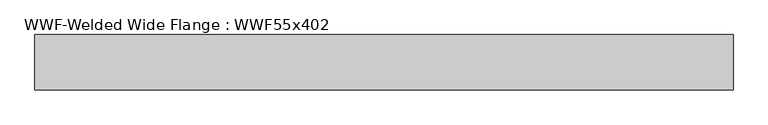
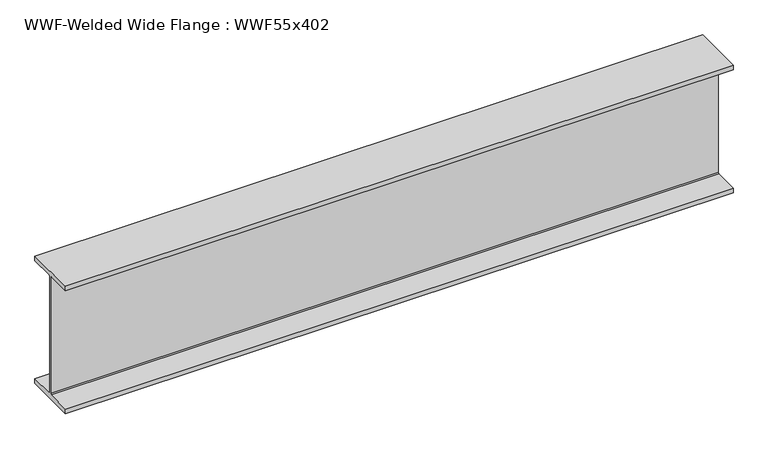
"""IFC4 building model written with IfcOpenShell, lengths in millimetres: beam geometry, WWF-Welded Wide Flange : WWF55x402."""

from ifc_helpers import new_model, si_unit, frame, origin, place, context, project, spatial, polyline, outline, extrude, source, transform, mapped, element, save


def wwf_welded_wide_flange_wwf55x402_453157a7(model_context):
    return source(origin(), model_context, "Body", "SweptSolid", [
        extrude(outline(polyline([(274.955, -649.986), (274.955, -700.024), (-274.955, -700.024), (-274.955, -649.986), (-19.05, -649.986), (-8.001, -638.937), (-8.001, 638.937), (-19.05, 649.986), (-274.955, 649.986), (-274.955, 700.024), (274.955, 700.024), (274.955, 649.986), (19.05, 649.986), (8.001, 638.937), (8.001, -638.937), (19.05, -649.986), (274.955, -649.986)])), frame((-3472.218169, 0.0, 0.0), z_axis=(1.0, 0.0, 0.0), x_axis=(0.0, 1.0, 0.0)), (0.0, 0.0, 1.0), 6944.436338),
    ])


if __name__ == "__main__":
    model = new_model("IFC4")
    model_context = context("Model", 3, world=origin())
    ifc_project = project(units=[si_unit("LENGTHUNIT", "METRE", prefix="MILLI")], contexts=[model_context])
    site = spatial("IfcSite", under=ifc_project)
    building = spatial("IfcBuilding", under=site)
    placement = place(None, origin())
    wwf_welded_wide_flange_wwf55x402_shape = wwf_welded_wide_flange_wwf55x402_453157a7(model_context)
    element("IfcBeam", 1, ObjectType="WWF-Welded Wide Flange : WWF55x402", at=placement, inside=building, context=model_context, shape_type="MappedRepresentation", body=[
        mapped(wwf_welded_wide_flange_wwf55x402_shape, transform((0.0, 0.0, 0.0), x_axis=(1.0, 0.0, 0.0), y_axis=(0.0, 1.0, 0.0), z_axis=(0.0, 0.0, 1.0))),
    ])
    save(model, "model.ifc")

# Revit data of these elements
# Type "WWF-Welded Wide Flange : WWF55x402"
#   Assembly Code = "B10"
#   Nominal d = "12"
#   W = 402
#   Length [instance default] = 1524 mm
#   bf = 549.91 mm
#   d = 1400.048 mm
#   k = 19.05 mm
#   tf = 50.038 mm
#   tw = 16.002 mm
#   A = 0.0761289 m²
#   Structural Material [instance default] = Steel ASTM A572
# Element 1 (IfcBeam, "WWF-Welded Wide Flange : WWF55x402")
#   Structural Material = Metal - Steel 43-275
#   Materials on its faces: "Metal - Steel 43-275"
# Materials
#   "Steel ASTM A572": class "Metal", colour RGB 247 247 247, transparency 0, Description = "Structural steel, high strength low alloy, ASTM - A572 - 50", Cost = 0
#   "Metal - Steel 43-275": class "Metal", colour RGB 247 247 247, transparency 0, Cost = 0
